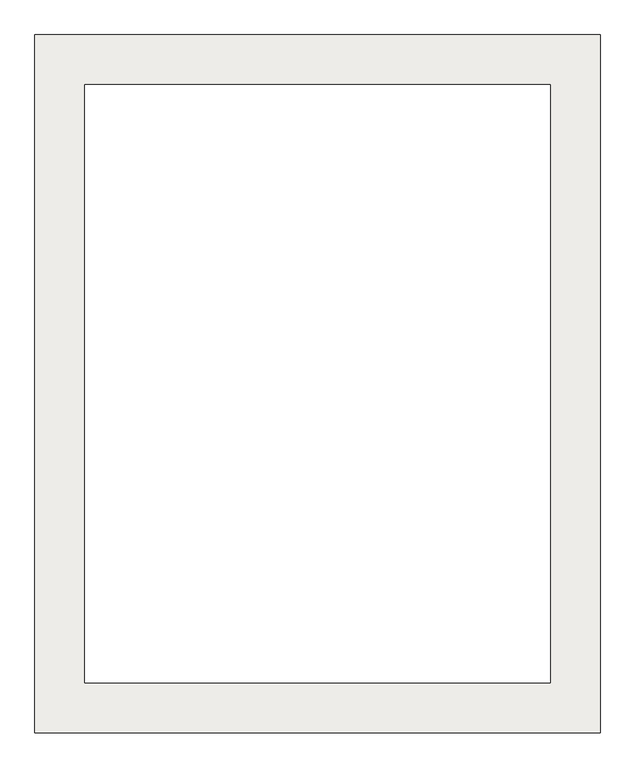
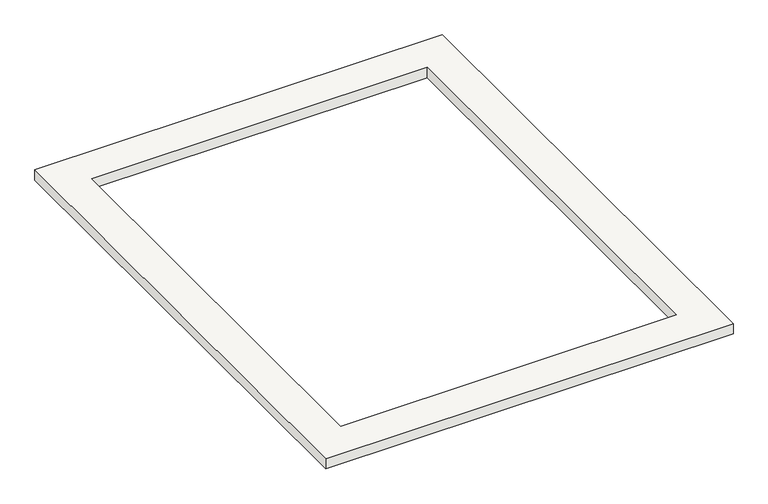
"""IFC4 building model written with IfcOpenShell, lengths in millimetres: slab geometry, Holzdecke."""

from ifc_helpers import new_model, si_unit, origin, origin_with_axes, place, context, project, spatial, polyline, outline, extrude, source, transform, mapped, element, save


def slab_def542f6(model_context):
    return source(origin(), model_context, "Body", "SweptSolid", [
        extrude(outline(polyline([(17000.0, 21002.8619019), (17000.0, 0.0), (0.0, 0.0), (0.0, 21002.8619019), (17000.0, 21002.8619019)]), holes=[polyline([(15500.0, 1500.0), (15500.0, 19502.8619019), (1500.0, 19502.8619019), (1500.0, 1500.0), (15500.0, 1500.0)])]), origin_with_axes(), (0.0, 0.0, 1.0), 450.0),
    ])


if __name__ == "__main__":
    model = new_model("IFC4")
    model_context = context("Model", 3, world=origin())
    ifc_project = project(units=[si_unit("LENGTHUNIT", "METRE", prefix="MILLI")], contexts=[model_context])
    site = spatial("IfcSite", under=ifc_project)
    building = spatial("IfcBuilding", under=site)
    placement = place(None, origin())
    slab_shape = slab_def542f6(model_context)
    element("IfcSlab", 1, ObjectType="Holzdecke", at=placement, inside=building, context=model_context, shape_type="MappedRepresentation", body=[
        mapped(slab_shape, transform((0.0, 0.0, 0.0), x_axis=(1.0, 0.0, 0.0), y_axis=(0.0, 1.0, 0.0), z_axis=(0.0, 0.0, 1.0))),
    ])
    save(model, "model.ifc")

# Revit data of these elements
# Element 1 (IfcSlab, "Holzdecke")
#   Materials on its faces: "holzschalung"
# Materials
#   "holzschalung": class "Unassigned", colour RGB 128 128 128, transparency 0
